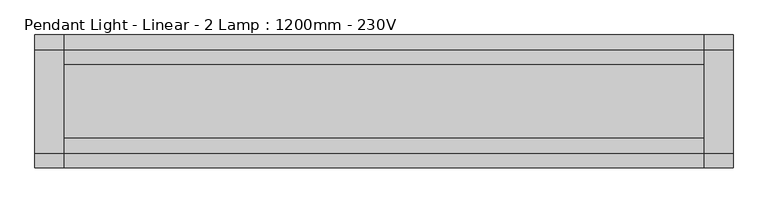
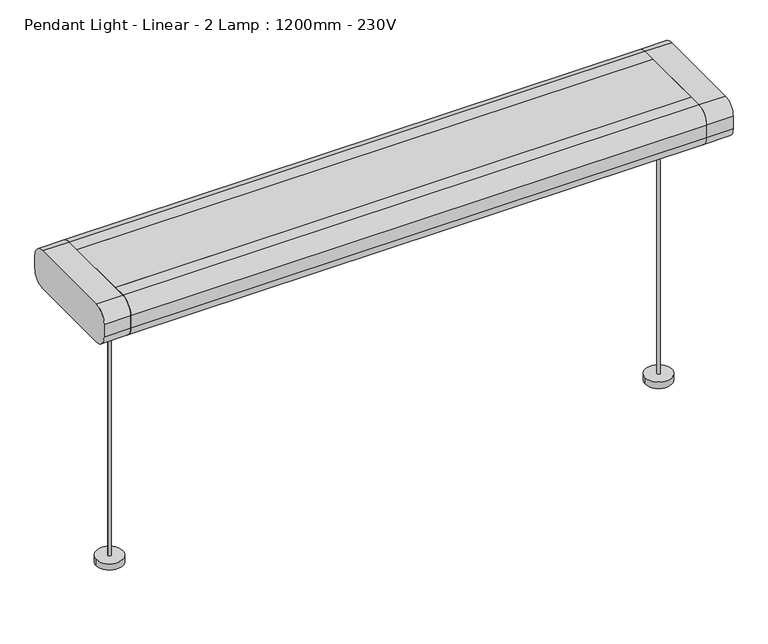
"""IFC4 building model written with IfcOpenShell, lengths in millimetres: light fixture geometry, Pendant Light - Linear - 2 Lamp : 1200mm - 230V."""

from ifc_helpers import new_model, si_unit, point, frame, frame_2d, origin, origin_with_axes, place, context, project, spatial, polyline, circle_curve, trimmed, segment, composite_curve, outline, extrude, source, transform, mapped, element, save


def pendant_light_linear_2_lamp_1200mm_230v_b97dd2e3(model_context):
    return source(origin(), model_context, "Body", "SweptSolid", [
        extrude(outline(composite_curve([segment(polyline([(114.3, 574.6), (114.3, 549.2)]), True, "CONTINUOUS"), segment(trimmed(circle_curve(frame_2d((88.9, 549.2)), 25.4), [point((114.3, 549.2))], [point((88.9, 523.8))], False, "CARTESIAN"), True, "CONTINUOUS"), segment(polyline([(88.9, 523.8), (-88.9, 523.8)]), True, "CONTINUOUS"), segment(trimmed(circle_curve(frame_2d((-88.9, 549.2)), 25.4), [point((-88.9, 523.8))], [point((-114.3, 549.2))], False, "CARTESIAN"), True, "CONTINUOUS"), segment(polyline([(-114.3, 549.2), (-114.3, 574.6)]), True, "CONTINUOUS"), segment(trimmed(circle_curve(frame_2d((-88.9, 574.6)), 25.4), [point((-114.3, 574.6))], [point((-88.9, 600.0))], False, "CARTESIAN"), True, "CONTINUOUS"), segment(polyline([(-88.9, 600.0), (-63.5, 600.0), (-63.5, 574.6), (63.5, 574.6), (63.5, 600.0), (88.9, 600.0)]), True, "CONTINUOUS"), segment(trimmed(circle_curve(frame_2d((88.9, 574.6)), 25.4), [point((88.9, 600.0))], [point((114.3, 574.6))], False, "CARTESIAN"), True, "CONTINUOUS")], self_intersect=False)), frame((-549.2, 0.0, 0.0), z_axis=(1.0, 0.0, 0.0), x_axis=(0.0, 1.0, 0.0)), (0.0, 0.0, 1.0), 1098.4),
        extrude(outline(polyline([(549.2, 63.5), (549.2, -63.5), (-549.2, -63.5), (-549.2, 63.5), (549.2, 63.5)])), frame((0.0, 0.0, 587.3), z_axis=(0.0, 0.0, 1.0), x_axis=(1.0, 0.0, 0.0)), (0.0, 0.0, 1.0), 12.7),
        extrude(outline(composite_curve([segment(trimmed(circle_curve(frame_2d((523.8, 0.0)), 25.4), [point((498.4, 0.0))], [point((549.2, 0.0))], False, "CARTESIAN"), True, "CONTINUOUS"), segment(trimmed(circle_curve(frame_2d((523.8, 0.0)), 25.4), [point((549.2, 0.0))], [point((498.4, 0.0))], False, "CARTESIAN"), True, "CONTINUOUS")], self_intersect=False)), origin_with_axes(), (0.0, 0.0, 1.0), 12.7),
        extrude(outline(composite_curve([segment(trimmed(circle_curve(frame_2d((-523.8, 0.0)), 25.4), [point((-549.2, 0.0))], [point((-498.4, 0.0))], False, "CARTESIAN"), True, "CONTINUOUS"), segment(trimmed(circle_curve(frame_2d((-523.8, 0.0)), 25.4), [point((-498.4, 0.0))], [point((-549.2, 0.0))], False, "CARTESIAN"), True, "CONTINUOUS")], self_intersect=False)), origin_with_axes(), (0.0, 0.0, 1.0), 12.7),
        extrude(outline(composite_curve([segment(trimmed(circle_curve(frame_2d((-88.9, 574.6)), 25.4), [point((-114.3, 574.6))], [point((-88.9, 600.0))], False, "CARTESIAN"), True, "CONTINUOUS"), segment(polyline([(-88.9, 600.0), (88.9, 600.0)]), True, "CONTINUOUS"), segment(trimmed(circle_curve(frame_2d((88.9, 574.6)), 25.4), [point((88.9, 600.0))], [point((114.3, 574.6))], False, "CARTESIAN"), True, "CONTINUOUS"), segment(polyline([(114.3, 574.6), (114.3, 549.2)]), True, "CONTINUOUS"), segment(trimmed(circle_curve(frame_2d((88.9, 549.2)), 25.4), [point((114.3, 549.2))], [point((88.9, 523.8))], False, "CARTESIAN"), True, "CONTINUOUS"), segment(polyline([(88.9, 523.8), (-88.9, 523.8)]), True, "CONTINUOUS"), segment(trimmed(circle_curve(frame_2d((-88.9, 549.2)), 25.4), [point((-88.9, 523.8))], [point((-114.3, 549.2))], False, "CARTESIAN"), True, "CONTINUOUS"), segment(polyline([(-114.3, 549.2), (-114.3, 574.6)]), True, "CONTINUOUS")], self_intersect=False)), frame((549.2, 0.0, 0.0), z_axis=(1.0, 0.0, 0.0), x_axis=(0.0, 1.0, 0.0)), (0.0, 0.0, 1.0), 50.8),
        extrude(outline(composite_curve([segment(polyline([(114.3, 574.6), (114.3, 549.2)]), True, "CONTINUOUS"), segment(trimmed(circle_curve(frame_2d((88.9, 549.2)), 25.4), [point((114.3, 549.2))], [point((88.9, 523.8))], False, "CARTESIAN"), True, "CONTINUOUS"), segment(polyline([(88.9, 523.8), (-88.9, 523.8)]), True, "CONTINUOUS"), segment(trimmed(circle_curve(frame_2d((-88.9, 549.2)), 25.4), [point((-88.9, 523.8))], [point((-114.3, 549.2))], False, "CARTESIAN"), True, "CONTINUOUS"), segment(polyline([(-114.3, 549.2), (-114.3, 574.6)]), True, "CONTINUOUS"), segment(trimmed(circle_curve(frame_2d((-88.9, 574.6)), 25.4), [point((-114.3, 574.6))], [point((-88.9, 600.0))], False, "CARTESIAN"), True, "CONTINUOUS"), segment(polyline([(-88.9, 600.0), (88.9, 600.0)]), True, "CONTINUOUS"), segment(trimmed(circle_curve(frame_2d((88.9, 574.6)), 25.4), [point((88.9, 600.0))], [point((114.3, 574.6))], False, "CARTESIAN"), True, "CONTINUOUS")], self_intersect=False)), frame((-600.0, 0.0, 0.0), z_axis=(1.0, 0.0, 0.0), x_axis=(0.0, 1.0, 0.0)), (0.0, 0.0, 1.0), 50.8),
        extrude(outline(composite_curve([segment(trimmed(circle_curve(frame_2d((523.8, 0.0)), 3.1340604), [point((520.6659396, 0.0))], [point((526.9340604, 0.0))], False, "CARTESIAN"), True, "CONTINUOUS"), segment(trimmed(circle_curve(frame_2d((523.8, 0.0)), 3.1340604), [point((526.9340604, 0.0))], [point((520.6659396, 0.0))], False, "CARTESIAN"), True, "CONTINUOUS")], self_intersect=False)), origin_with_axes(), (0.0, 0.0, 1.0), 523.8),
        extrude(outline(composite_curve([segment(trimmed(circle_curve(frame_2d((-523.8, 0.0)), 3.175), [point((-526.975, 0.0))], [point((-520.625, 0.0))], False, "CARTESIAN"), True, "CONTINUOUS"), segment(trimmed(circle_curve(frame_2d((-523.8, 0.0)), 3.175), [point((-520.625, 0.0))], [point((-526.975, 0.0))], False, "CARTESIAN"), True, "CONTINUOUS")], self_intersect=False)), origin_with_axes(), (0.0, 0.0, 1.0), 523.8),
    ])


if __name__ == "__main__":
    model = new_model("IFC4")
    model_context = context("Model", 3, world=origin())
    ifc_project = project(units=[si_unit("LENGTHUNIT", "METRE", prefix="MILLI")], contexts=[model_context])
    site = spatial("IfcSite", under=ifc_project)
    building = spatial("IfcBuilding", under=site)
    placement = place(None, origin())
    pendant_light_linear_2_lamp_1200mm_230v_shape = pendant_light_linear_2_lamp_1200mm_230v_b97dd2e3(model_context)
    element("IfcLightFixture", 1, ObjectType="Pendant Light - Linear - 2 Lamp : 1200mm - 230V", at=placement, inside=building, context=model_context, shape_type="MappedRepresentation", body=[
        mapped(pendant_light_linear_2_lamp_1200mm_230v_shape, transform((0.0, 0.0, 0.0), x_axis=(1.0, 0.0, 0.0), y_axis=(0.0, 1.0, 0.0), z_axis=(0.0, 0.0, 1.0))),
    ])
    save(model, "model.ifc")

# Revit data of these elements
# Type "Pendant Light - Linear - 2 Lamp : 1200mm - 230V"
#   Type Mark = "Pendant Light - Linear - 2 Lamp"
#   Classification.OmniClass.23.Number = "23-35 47 11"
#   Classification.OmniClass.23.Description = "Lighting Fixtures"
#   COBie.Type.CreatedBy = "info@mma.ie"
#   COBie.Type.CreatedOn = "2017-07-25T10:15:16"
#   COBie.Type.Name = "Pendant Light - Linear - 2 Lamp"
#   COBie.Type.Category = "23-35 47 11 : Lighting Fixtures"
#   COBie.Type.Description = "Pendant Light - Linear - 2 Lamp_1200mm - 230V"
#   COBie.Type.AssetType = "Fixed"
#   COBie.Type.Manufacturer = ""
#   COBie.Type.ModelNumber = ""
#   Photometric Web File = "482T12.ies"
#   Lamp = "T-12"
#   Keynote = "26 51 00.A"
#   Assembly Code = "D5020210"
#   COBie.Type.ReplacementCost = 0
#   Wattage = 64 W
#   built-in parameter 1150110 = 1 (stored number, unit not read)
#   built-in parameter 1150109 = 1 (stored number, unit not read)
#   built-in parameter 1150113 = 1 (stored number, unit not read)
#   Tilt Angle = -90.00°
#   P.L. Width = 228.6 mm
#   P.L. Length = 1200 mm
#   P.L. Drop from Ceiling = 600 mm
#   Lumens = 6000 lm
#   built-in parameter 1114217 = 0.88 (stored number, unit not read)
#   built-in parameter 1150115 = 1 (stored number, unit not read)
#   built-in parameter 1150105 = 477.465 (stored number, unit not read)
#   Light Casing Length = 1200 mm
#   built-in parameter 1150112 = 1 (stored number, unit not read)
#   built-in parameter 1150114 = 1 (stored number, unit not read)
#   built-in parameter 1150107 = 4230 (stored number, unit not read)
#   built-in parameter 1150106 = 4.77465 (stored number, unit not read)
#   Emit from Rectangle Width = 127.6 mm
#   Emit from Rectangle Length = 1098 mm
#   built-in parameter 1150104 = 8.70966 (stored number, unit not read)
#   Drop From Ceiling = 600 mm
#   Default Elevation = 1200 mm
#   Ballast Voltage = 230 V
#   built-in parameter 1114218 = 0.88 (stored number, unit not read)
#   built-in parameter 1150133 = 10 (stored number, unit not read)
#   Apparent Load = 64 VA
#   COBie.Type = yes
#   built-in parameter 1150134 = 8
#   built-in parameter 1150137 = 1
#   Color Filter = 16777215
#   built-in parameter 1140040 [instance default] = 1
#   Ballast Number of Poles = 1
#   Load Classification = Lighting - Dwelling Unit
#   Light Casing Material = Metal - Paint Finish - Ivory, Glossy
#   Diffuser Material = Glass - White, High Luminance
#   Ceiling Mount Material = Metal - Paint Finish - Ivory, Glossy
#   Emit Shape Visible in Rendering = no
#   Dimming Lamp Color Temperature Shift = (empty or 0)
# Element 1 (IfcLightFixture, "Pendant Light - Linear - 2 Lamp : 1200mm - 230V")
#   Materials on its faces: "Metal - Paint Finish - Ivory, Glossy", "Glass - White, High Luminance"
# Materials
#   "Metal - Paint Finish - Ivory, Glossy": class "Paint", colour RGB 247 247 239, transparency 0, Comments = "Rendering appearance not upgraded "
#   "Glass - White, High Luminance": class "Glass", colour RGB 249 250 249, transparency 0.8
